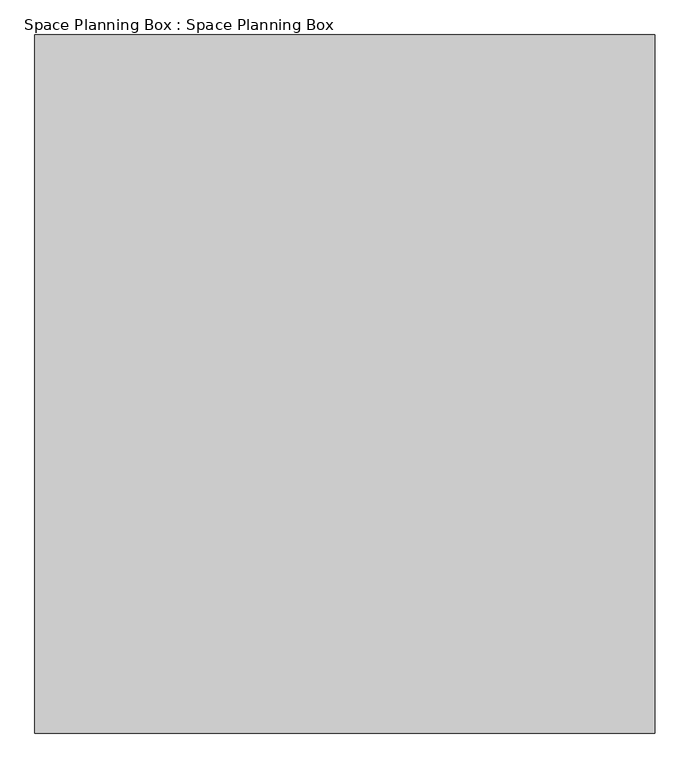
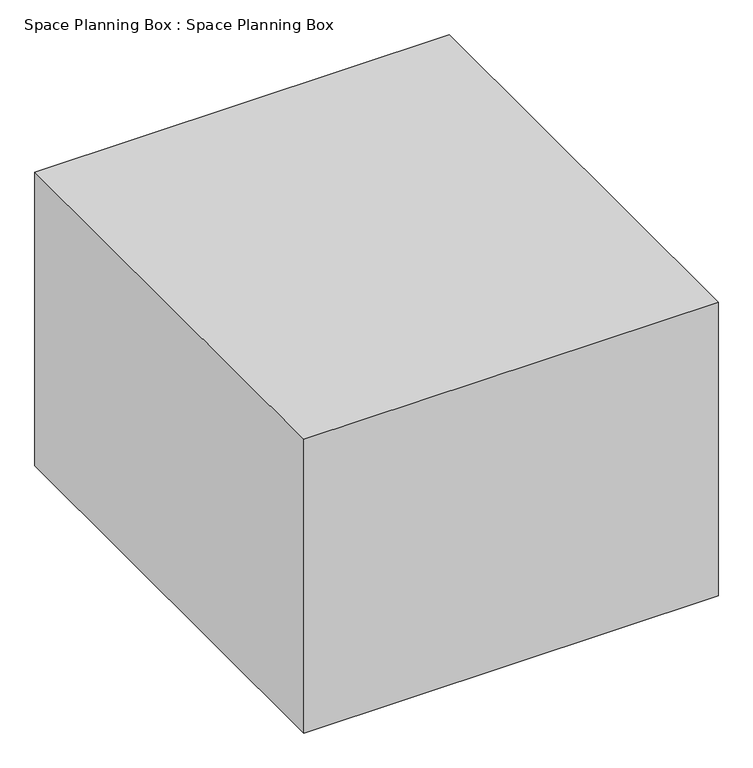
"""IFC4 building model written with IfcOpenShell, lengths in millimetres: proxy geometry, Space Planning Box : Space Planning Box."""

import ifcopenshell
import ifcopenshell.guid

model = None  # the IFC model being written
_history = None  # IfcOwnerHistory: only IFC2X3 demands one
_inside = {}  # id of a spatial element -> (the spatial element, [elements in it])
_under = {}  # id of a project, library or spatial element -> (it, [spatial elements below it])
_declared = {}  # id of a project -> (the project, [libraries it declares])
_typed = {}  # id of a type object -> (the type object, [elements of that type])
_made_of = {}  # id of a material, layer set ... -> (it, [elements and type objects made of it])


def new_model(schema):
    """Start an empty IFC model of exactly this schema.

    Asked for "IFC4X3", IfcOpenShell would pick the latest addendum, in which some entities
    have other attributes; the version numbers below select the first issue.
    IFC2X3 requires an IfcOwnerHistory on every rooted entity: one is made here for all.
    """
    global model, _history
    if schema == "IFC4X3":
        model = ifcopenshell.file(schema_version=(4, 3, 0, 0))
    else:
        model = ifcopenshell.file(schema=schema)
    _inside.clear()
    _under.clear()
    _declared.clear()
    _typed.clear()
    _made_of.clear()
    _history = None
    if model.schema == "IFC2X3":
        org = make("IfcOrganization", Name="unknown")
        user = make(
            "IfcPersonAndOrganization",
            ThePerson=make("IfcPerson", FamilyName="unknown"),
            TheOrganization=org,
        )
        app = make(
            "IfcApplication",
            ApplicationDeveloper=org,
            Version="unknown",
            ApplicationFullName="unknown",
            ApplicationIdentifier="unknown",
        )
        _history = make(
            "IfcOwnerHistory",
            OwningUser=user,
            OwningApplication=app,
            ChangeAction="ADDED",
            CreationDate=0,
        )
    return model


def make(cls, **values):
    """One entity of the class cls with the attributes given. An attribute that is None is left unset."""
    return model.create_entity(
        cls, **{name: value for name, value in values.items() if value is not None}
    )


def rooted(cls, **values):
    """An entity with a GlobalId (a new one), such as an element, a storey or a relation."""
    return make(cls, GlobalId=ifcopenshell.guid.new(), OwnerHistory=_history, **values)


def si_unit(unit_type, name, prefix=None):
    """IfcSIUnit, for example si_unit("LENGTHUNIT", "METRE", prefix="MILLI")."""
    return make("IfcSIUnit", UnitType=unit_type, Prefix=prefix, Name=name)


def assignment(units):
    """IfcUnitAssignment: the units of a project."""
    return None if units is None else make("IfcUnitAssignment", Units=units)


def point(xyz):
    """IfcCartesianPoint."""
    return None if xyz is None else make("IfcCartesianPoint", Coordinates=xyz)


def direction(xyz):
    """IfcDirection."""
    return None if xyz is None else make("IfcDirection", DirectionRatios=xyz)


def frame(location, z_axis=None, x_axis=None):
    """IfcAxis2Placement3D, a coordinate frame: its origin and axes. An axis left out is left unset."""
    return make(
        "IfcAxis2Placement3D",
        Location=point(location),
        Axis=direction(z_axis),
        RefDirection=direction(x_axis),
    )


def origin():
    """The frame at (0, 0, 0) with its axes left unset."""
    return frame((0.0, 0.0, 0.0))


def origin_with_axes():
    """The frame at (0, 0, 0) with the z axis (0, 0, 1) and the x axis (1, 0, 0) written out."""
    return frame((0.0, 0.0, 0.0), z_axis=(0.0, 0.0, 1.0), x_axis=(1.0, 0.0, 0.0))


def place(relative_to, where):
    """IfcLocalPlacement: puts the frame where relative to a parent placement (None: the world)."""
    return make(
        "IfcLocalPlacement", PlacementRelTo=relative_to, RelativePlacement=where
    )


def context(
    kind, dimensions, precision=None, world=None, true_north=None, identifier=None
):
    """IfcGeometricRepresentationContext, for example the 3D "Model" context."""
    return make(
        "IfcGeometricRepresentationContext",
        ContextIdentifier=identifier,
        ContextType=kind,
        CoordinateSpaceDimension=dimensions,
        Precision=precision,
        WorldCoordinateSystem=world,
        TrueNorth=true_north,
    )


def project(units=None, contexts=None):
    """IfcProject with its units and contexts."""
    return rooted(
        "IfcProject",
        Name="project",
        RepresentationContexts=contexts,
        UnitsInContext=assignment(units),
    )


def spatial(cls, under=None, at=None, **own):
    """A site, building, storey or space (cls), placed at a placement, below another one or the project."""
    s = rooted(cls, ObjectPlacement=at, **own)
    if under is not None:
        _under.setdefault(under.id(), (under, []))[1].append(s)
    return s


def polyline(points):
    """IfcPolyline through the points."""
    return make("IfcPolyline", Points=[point(p) for p in points])


def outline(outer, holes=None, kind="AREA"):
    """IfcArbitraryClosedProfileDef: a profile drawn as a closed curve; with holes, ...WithVoids."""
    if holes is None:
        return make("IfcArbitraryClosedProfileDef", ProfileType=kind, OuterCurve=outer)
    return make(
        "IfcArbitraryProfileDefWithVoids",
        ProfileType=kind,
        OuterCurve=outer,
        InnerCurves=holes,
    )


def extrude(swept, where, along, depth):
    """IfcExtrudedAreaSolid: the profile swept, set in the frame where, extruded along a direction by depth."""
    return make(
        "IfcExtrudedAreaSolid",
        SweptArea=swept,
        Position=where,
        ExtrudedDirection=direction(along),
        Depth=depth,
    )


def shape(context_of_items, identifier, shape_type, items):
    """IfcShapeRepresentation: the items that make up one representation, for example the "Body"."""
    return make(
        "IfcShapeRepresentation",
        ContextOfItems=context_of_items,
        RepresentationIdentifier=identifier,
        RepresentationType=shape_type,
        Items=items,
    )


def source(mapping_origin, context_of_items, identifier, shape_type, items):
    """IfcRepresentationMap: a shape defined once, which mapped items show again and again."""
    return make(
        "IfcRepresentationMap",
        MappingOrigin=mapping_origin,
        MappedRepresentation=shape(context_of_items, identifier, shape_type, items),
    )


def transform(
    local_origin,
    x_axis=None,
    y_axis=None,
    z_axis=None,
    scale=None,
    scale2=None,
    scale3=None,
    uniform=True,
):
    """IfcCartesianTransformationOperator3D, or its non-uniform kind. x_axis, y_axis, z_axis: its Axis1, 2, 3."""
    if uniform:
        return make(
            "IfcCartesianTransformationOperator3D",
            Axis1=direction(x_axis),
            Axis2=direction(y_axis),
            LocalOrigin=point(local_origin),
            Scale=scale,
            Axis3=direction(z_axis),
        )
    return make(
        "IfcCartesianTransformationOperator3DnonUniform",
        Axis1=direction(x_axis),
        Axis2=direction(y_axis),
        LocalOrigin=point(local_origin),
        Scale=scale,
        Axis3=direction(z_axis),
        Scale2=scale2,
        Scale3=scale3,
    )


def mapped(mapping_source, mapping_target):
    """IfcMappedItem: shows the shape of a source again, moved by a transform."""
    return make(
        "IfcMappedItem", MappingSource=mapping_source, MappingTarget=mapping_target
    )


def made_of(thing, what):
    """Note that an element or type object is made of a material, layer set ...; save() writes the relation."""
    if what is not None:
        _made_of.setdefault(what.id(), (what, []))[1].append(thing)
    return thing


def element(
    cls,
    number,
    at=None,
    inside=None,
    cuts=None,
    type_object=None,
    material=None,
    context=None,
    identifier="Body",
    shape_type=None,
    held_by="IfcProductDefinitionShape",
    body=None,
    shapes=None,
    **own,
):
    """One element of the class cls, such as IfcWall. Its Tag is "e" and its number.

    at: its placement. inside: the storey or other place that contains it. cuts: it is an
    opening in that element (IfcRelVoidsElement). A single representation is given by context,
    identifier, shape_type and body (its items); several are given by shapes. held_by: the class
    of the entity that holds the representations. save() writes the other relations.
    """
    e = rooted(cls, Tag="e%d" % number, ObjectPlacement=at, **own)
    if body is not None:
        shapes = [shape(context, identifier, shape_type, body)]
    if shapes is not None:
        e.Representation = make(held_by, Representations=shapes)
    if inside is not None:
        _inside.setdefault(inside.id(), (inside, []))[1].append(e)
    if cuts is not None:
        rooted(
            "IfcRelVoidsElement", RelatingBuildingElement=cuts, RelatedOpeningElement=e
        )
    if type_object is not None:
        _typed.setdefault(type_object.id(), (type_object, []))[1].append(e)
    return made_of(e, material)


def aggregate(whole, parts):
    """IfcRelAggregates: a whole, such as a stair, and the parts it consists of."""
    return rooted("IfcRelAggregates", RelatingObject=whole, RelatedObjects=parts)


def save(model, path):
    """Write the relations noted so far, then the file.

    IfcRelAggregates (storeys below a building ...), IfcRelContainedInSpatialStructure (elements
    in a storey), IfcRelDefinesByType, IfcRelAssociatesMaterial and IfcRelDeclares: one each for
    every whole, place, type object, material and project.
    """
    for whole, parts in _under.values():
        aggregate(whole, parts)
    for where, things in _inside.values():
        rooted(
            "IfcRelContainedInSpatialStructure",
            RelatedElements=things,
            RelatingStructure=where,
        )
    for kind, things in _typed.values():
        rooted("IfcRelDefinesByType", RelatedObjects=things, RelatingType=kind)
    for what, things in _made_of.values():
        rooted("IfcRelAssociatesMaterial", RelatedObjects=things, RelatingMaterial=what)
    for by, libraries in _declared.values():
        rooted("IfcRelDeclares", RelatingContext=by, RelatedDefinitions=libraries)
    model.write(path)


def space_planning_box_space_planning_box_4d084078(model_context):
    return source(origin(), model_context, "Body", "SweptSolid", [
        extrude(outline(polyline([(4000.0, 4500.0), (4000.0, -4500.0), (-4000.0, -4500.0), (-4000.0, 4500.0), (4000.0, 4500.0)])), origin_with_axes(), (0.0, 0.0, 1.0), 6000.0),
    ])


if __name__ == "__main__":
    model = new_model("IFC4")
    model_context = context("Model", 3, world=origin())
    ifc_project = project(units=[si_unit("LENGTHUNIT", "METRE", prefix="MILLI")], contexts=[model_context])
    site = spatial("IfcSite", under=ifc_project)
    building = spatial("IfcBuilding", under=site)
    placement = place(None, origin())
    space_planning_box_space_planning_box_shape = space_planning_box_space_planning_box_4d084078(model_context)
    element("IfcBuildingElementProxy", 1, Name="Space Planning Box : Space Planning Box", ObjectType="Space Planning Box : Space Planning Box", at=placement, inside=building, context=model_context, shape_type="MappedRepresentation", body=[
        mapped(space_planning_box_space_planning_box_shape, transform((0.0, 0.0, 0.0), x_axis=(1.0, 0.0, 0.0), y_axis=(0.0, 1.0, 0.0), z_axis=(0.0, 0.0, 1.0))),
    ])
    save(model, "model.ifc")

# Revit data of these elements
# Project information
#   Project Issue Date = "Issue Date"
#   Project Status = "Project Status"
#   Client Name = "Owner"
#   Project Address = "Enter address here"
#   Project Name = "Project Name"
#   Project Number = "Project Number"
# Type "Space Planning Box : Space Planning Box"
#   Type Comments = "..."
#   Room Name [instance default] = "?"
#   Assembly Code = "..."
#   Width [instance default] = 1524 mm
#   Program Area [instance default] = 0 m²
#   Length [instance default] = 1524 mm
#   Height [instance default] = 1524 mm
#   Area [instance default] = 2.32258 m²
#   Fill Color [instance default] = Cyan
#   Default Elevation = 0
# Element 1 (IfcBuildingElementProxy, "Space Planning Box : Space Planning Box")
#   Room Name = "Fire Gas Room"
#   Width = 8000 mm
#   Length = 9000 mm
#   Height = 6000 mm
#   Area = 72 m²
#   Materials on its faces: "Cyan"
# Materials
#   "Cyan": class "Generic", colour RGB 0 255 255, transparency 0.2, Cost = 0
